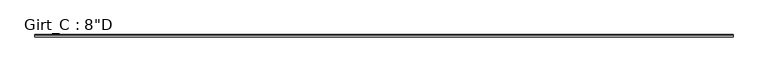
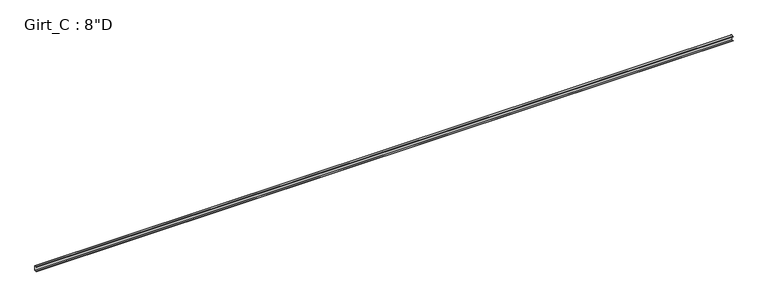
"""IFC4 building model written with IfcOpenShell, lengths in millimetres: beam geometry."""

from ifc_helpers import new_model, si_unit, point, frame, frame_2d, origin, place, context, project, spatial, polyline, circle_curve, trimmed, segment, composite_curve, outline, extrude, source, transform, mapped, element, save


def beam_88a5fd93(model_context):
    return source(origin(), model_context, "Body", "SweptSolid", [
        extrude(outline(composite_curve([segment(polyline([(-87.5109375, 101.6), (-3.3734375, 101.6)]), True, "CONTINUOUS"), segment(trimmed(circle_curve(frame_2d((-3.3734375, 96.8375)), 4.7625), [point((-3.3734375, 101.6))], [point((1.3890625, 96.8375))], False, "CARTESIAN"), True, "CONTINUOUS"), segment(polyline([(1.3890625, 96.8375), (1.3890625, -96.8375)]), True, "CONTINUOUS"), segment(trimmed(circle_curve(frame_2d((-3.3734375, -96.8375)), 4.7625), [point((1.3890625, -96.8375))], [point((-3.3734375, -101.6))], False, "CARTESIAN"), True, "CONTINUOUS"), segment(polyline([(-3.3734375, -101.6), (-87.5109375, -101.6), (-99.7792647, -86.979177), (-97.6510975, -85.1934327), (-86.2154765, -98.821875), (-3.2694106, -98.821875)]), True, "CONTINUOUS"), segment(trimmed(circle_curve(frame_2d((-3.3748024, -96.8389339)), 1.9857399), [point((-3.2694106, -98.821875))], [point((-1.3890625, -96.8389339))], True, "CARTESIAN"), True, "CONTINUOUS"), segment(polyline([(-1.3890625, -96.8389339), (-1.3890625, 96.8381931)]), True, "CONTINUOUS"), segment(trimmed(circle_curve(frame_2d((-3.3741066, 96.8381931)), 1.9850441), [point((-1.3890625, 96.8381931))], [point((-3.3005807, 98.821875))], True, "CARTESIAN"), True, "CONTINUOUS"), segment(polyline([(-3.3005807, 98.821875), (-86.2154765, 98.821875), (-97.6278742, 85.221109), (-99.7560415, 87.0068534), (-87.5109375, 101.6)]), True, "CONTINUOUS")], self_intersect=False)), frame((-14148.6100916, 0.0, 0.0), z_axis=(1.0, 0.0, 0.0), x_axis=(0.0, 1.0, 0.0)), (0.0, 0.0, 1.0), 28297.2201833),
    ])


if __name__ == "__main__":
    model = new_model("IFC4")
    model_context = context("Model", 3, world=origin())
    ifc_project = project(units=[si_unit("LENGTHUNIT", "METRE", prefix="MILLI")], contexts=[model_context])
    site = spatial("IfcSite", under=ifc_project)
    building = spatial("IfcBuilding", under=site)
    placement = place(None, origin())
    beam_shape = beam_88a5fd93(model_context)
    element("IfcBeam", 1, ObjectType="Girt_C : 8\"D", at=placement, inside=building, context=model_context, shape_type="MappedRepresentation", body=[
        mapped(beam_shape, transform((0.0, 0.0, 0.0), x_axis=(1.0, 0.0, 0.0), y_axis=(0.0, 1.0, 0.0), z_axis=(0.0, 0.0, 1.0))),
    ])
    save(model, "model.ifc")

# Revit data of these elements
# Type "Girt_C : 8\"D"
#   half leg = 0' - 1 3/4"
#   Web_Thickness = 0' - 0 7/64"
#   Length [instance default] = 10' - 0"
#   Leg_1 = 0' - 3 1/2"
#   Height = 0' - 8"
#   Structural Material [instance default] = none
# Element 1 (IfcBeam, "Girt_C : 8\"D")
#   Structural Material = CEE' SECTION (8.0x3.5C - SEE STRUCT. DWGS)
#   Materials on its faces: "CEE' SECTION (8.0x3.5C - SEE STRUCT. DWGS)"
# Materials
#   "CEE' SECTION (8.0x3.5C - SEE STRUCT. DWGS)": class "Metal", colour RGB 137 146 153, transparency 0, Description = "Steel, mill finish", Cost = 0
